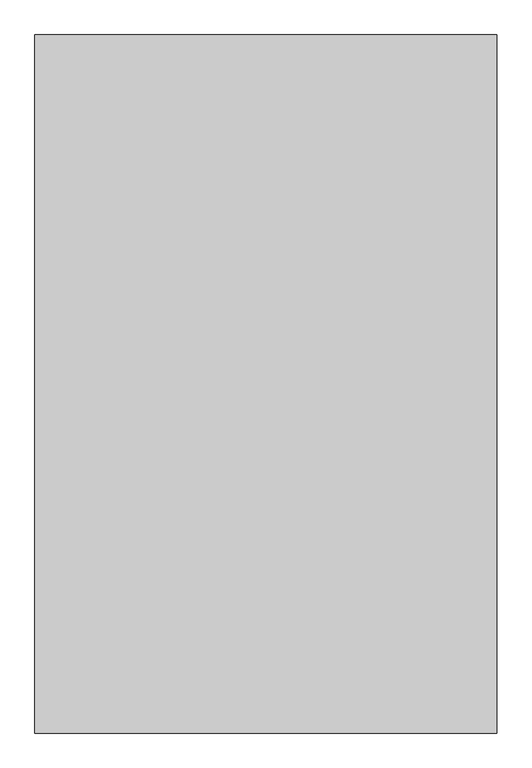
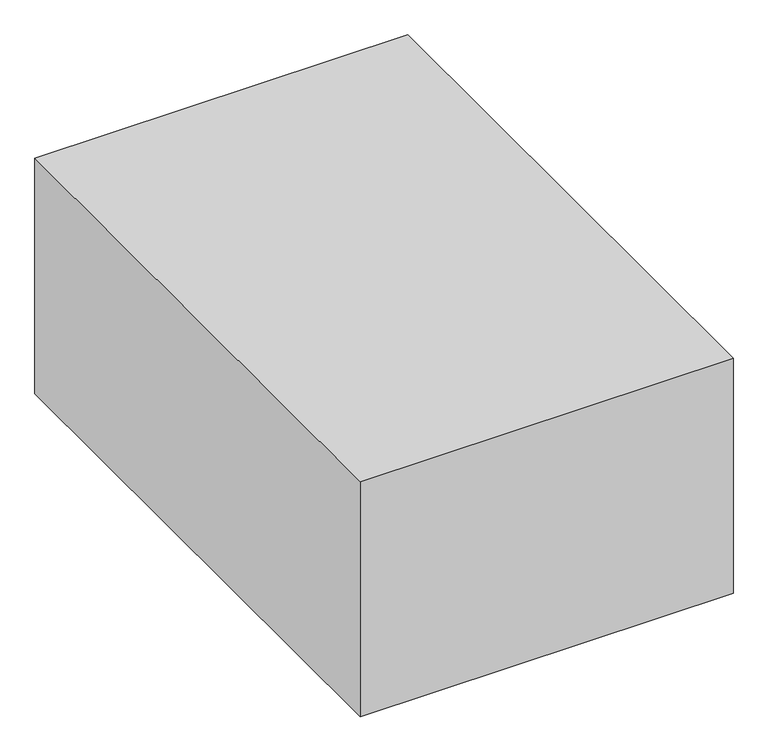
"""IFC4 building model written with IfcOpenShell, lengths in millimetres: proxy geometry, Space Planning Box_hec : Space Planning Box_hec."""

from ifc_helpers import new_model, si_unit, origin, origin_with_axes, place, context, project, spatial, polyline, outline, extrude, source, transform, mapped, element, save


def generic_models_af0009da(model_context):
    return source(origin(), model_context, "Body", "SweptSolid", [
        extrude(outline(polyline([(4500.0, 6800.0), (4500.0, -6800.0), (-4500.0, -6800.0), (-4500.0, 6800.0), (4500.0, 6800.0)])), origin_with_axes(), (0.0, 0.0, 1.0), 6000.0),
    ])


if __name__ == "__main__":
    model = new_model("IFC4")
    model_context = context("Model", 3, world=origin())
    ifc_project = project(units=[si_unit("LENGTHUNIT", "METRE", prefix="MILLI")], contexts=[model_context])
    site = spatial("IfcSite", under=ifc_project)
    building = spatial("IfcBuilding", under=site)
    placement = place(None, origin())
    generic_models_shape = generic_models_af0009da(model_context)
    element("IfcBuildingElementProxy", 1, Name="Space Planning Box_hec : Space Planning Box_hec", ObjectType="Space Planning Box_hec : Space Planning Box_hec", at=placement, inside=building, context=model_context, shape_type="MappedRepresentation", body=[
        mapped(generic_models_shape, transform((0.0, 0.0, 0.0), x_axis=(1.0, 0.0, 0.0), y_axis=(0.0, 1.0, 0.0), z_axis=(0.0, 0.0, 1.0))),
    ])
    save(model, "model.ifc")

# Revit data of these elements
# Type "Space Planning Box_hec : Space Planning Box_hec"
#   Type Comments = "..."
#   Room Name [instance default] = "?"
#   Interior Finish [instance default] = ""
#   Exterior Finish [instance default] = ""
#   Department [instance default] = ""
#   Assembly Code = "..."
#   Width [instance default] = 1524 mm
#   Program Area [instance default] = 0 m²
#   Length [instance default] = 1524 mm
#   Height [instance default] = 1524 mm
#   Area [instance default] = 2.32258 m²
#   Fill Color [instance default] = Cyan
#   Default Elevation = 0
# Element 1 (IfcBuildingElementProxy, "Space Planning Box_hec : Space Planning Box_hec")
#   Room Name = "Engineer Room"
#   Interior Finish = "IF3"
#   Exterior Finish = "EF1"
#   Department = "CI"
#   Width = 9000 mm
#   Program Area = 120 m²
#   Length = 13600 mm
#   Height = 6000 mm
#   Area = 122.4 m²
#   Fill Color = Lime
#   Materials on its faces: "Lime"
# Materials
#   "Cyan": class "Generic", colour RGB 0 255 255, transparency 0.2, Cost = 0
#   "Lime": class "Generic", colour RGB 0 255 0, transparency 0.2, Cost = 0
